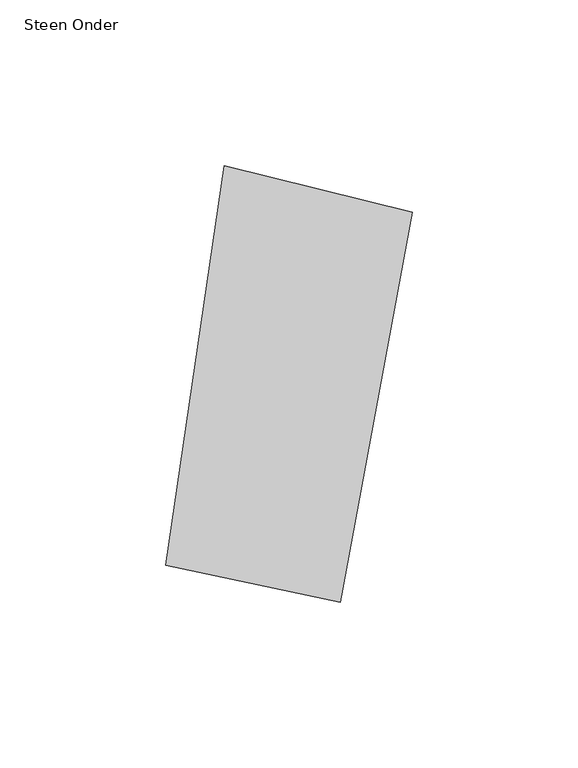
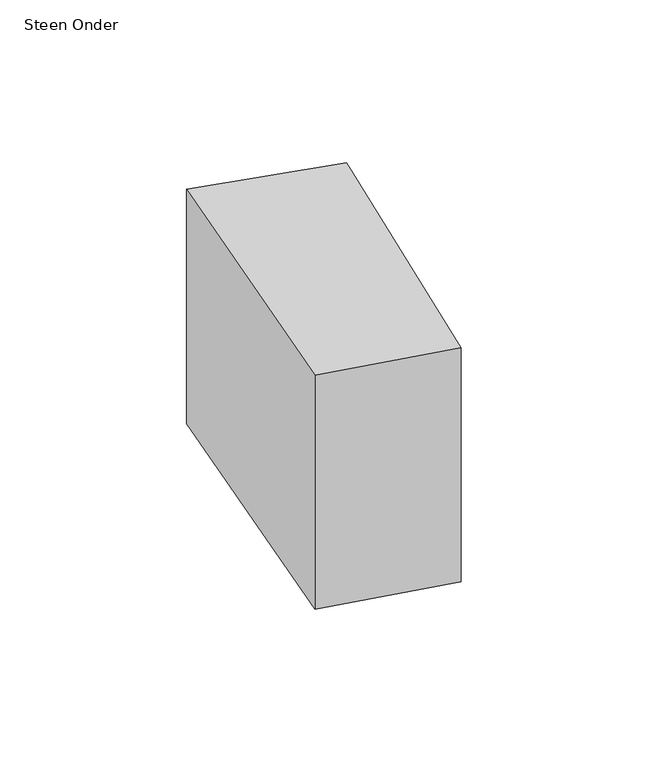
"""IFC4 building model written with IfcOpenShell, lengths in millimetres: proxy geometry, 00_GMA_steen_versie_4 : Steen Onder."""

from ifc_helpers import new_model, si_unit, origin, origin_with_axes, place, context, project, spatial, polyline, outline, extrude, source, transform, mapped, element, save


def steen_onder_56653986(model_context):
    return source(origin(), model_context, "Body", "SweptSolid", [
        extrude(outline(polyline([(111.1486147, 126.2754385), (89.3761678, 8.5685134), (36.8075119, 19.7051924), (54.4563267, 140.2333883), (111.1486147, 126.2754385)])), origin_with_axes(), (0.0, 0.0, 1.0), 100.0),
    ])


if __name__ == "__main__":
    model = new_model("IFC4")
    model_context = context("Model", 3, world=origin())
    ifc_project = project(units=[si_unit("LENGTHUNIT", "METRE", prefix="MILLI")], contexts=[model_context])
    site = spatial("IfcSite", under=ifc_project)
    building = spatial("IfcBuilding", under=site)
    placement = place(None, origin())
    steen_onder_shape = steen_onder_56653986(model_context)
    element("IfcBuildingElementProxy", 1, Name="00_GMA_steen_versie_4 : Steen Onder", ObjectType="00_GMA_steen_versie_4 : Steen Onder", at=placement, inside=building, context=model_context, shape_type="MappedRepresentation", body=[
        mapped(steen_onder_shape, transform((0.0, 0.0, 0.0), x_axis=(1.0, 0.0, 0.0), y_axis=(0.0, 1.0, 0.0), z_axis=(0.0, 0.0, 1.0))),
    ])
    save(model, "model.ifc")

# Revit data of these elements
# Type "00_GMA_steen_versie_4 : Steen Onder"
#   StootVoegHalfBoven [instance default] = 5 mm
#   StootVoegHalf [instance default] = 5 mm
#   StootVoegBreedteOnder = 10 mm
#   StootVoegBreedteBoven = 10 mm
#   Steendikte = 100 mm
#   LintVoegOnderHalf = 0 mm
#   LintVoegOnder = 0 mm
#   LintVoegBovenHalf = 5 mm
#   LintVoegBoven = 10 mm
#   materiaal = none
#   MateriaalVoeg = none
#   Default Elevation = 0
